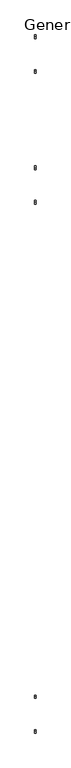
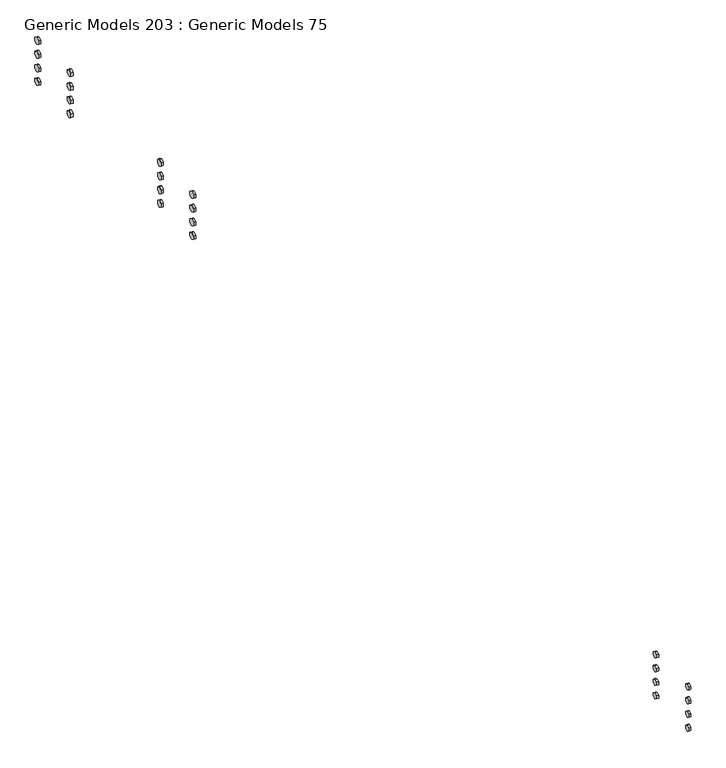
"""IFC4 building model written with IfcOpenShell, lengths in millimetres: proxy geometry, Generic Models 203 : Generic Models 75."""

from ifc_helpers import new_model, si_unit, frame, origin, place, context, project, spatial, polyline, outline, extrude, source, transform, mapped, element, save


def generic_models_203_generic_models_75_2103832a(model_context):
    return source(origin(), model_context, "Body", "SweptSolid", [
        extrude(outline(polyline([(30612.3964892, 271527.9099609), (30626.7031612, 271536.1699219), (30641.0098332, 271527.9099609), (30641.0098332, 271511.3900391), (30626.7031612, 271503.1300781), (30612.3964892, 271511.3900391), (30612.3964892, 271527.9099609)])), frame((31930.9715778, 0.0, 0.0), z_axis=(1.0, 0.0, 0.0), x_axis=(0.0, 1.0, 0.0)), (0.0, 0.0, 1.0), 11.90625),
        extrude(outline(polyline([(30612.3964892, 271604.1099609), (30626.7031612, 271612.3699219), (30641.0098332, 271604.1099609), (30641.0098332, 271587.5900391), (30626.7031612, 271579.3300781), (30612.3964892, 271587.5900391), (30612.3964892, 271604.1099609)])), frame((31930.9715778, 0.0, 0.0), z_axis=(1.0, 0.0, 0.0), x_axis=(0.0, 1.0, 0.0)), (0.0, 0.0, 1.0), 11.90625),
        extrude(outline(polyline([(30612.3964892, 271680.3099609), (30626.7031612, 271688.5699219), (30641.0098332, 271680.3099609), (30641.0098332, 271663.7900391), (30626.7031612, 271655.5300781), (30612.3964892, 271663.7900391), (30612.3964892, 271680.3099609)])), frame((31930.9715778, 0.0, 0.0), z_axis=(1.0, 0.0, 0.0), x_axis=(0.0, 1.0, 0.0)), (0.0, 0.0, 1.0), 11.90625),
        extrude(outline(polyline([(30612.3964892, 271756.5099609), (30626.7031612, 271764.7699219), (30641.0098332, 271756.5099609), (30641.0098332, 271739.9900391), (30626.7031612, 271731.7300781), (30612.3964892, 271739.9900391), (30612.3964892, 271756.5099609)])), frame((31930.9715778, 0.0, 0.0), z_axis=(1.0, 0.0, 0.0), x_axis=(0.0, 1.0, 0.0)), (0.0, 0.0, 1.0), 11.90625),
        extrude(outline(polyline([(30907.6714892, 271527.9099609), (30921.9781612, 271536.1699219), (30936.2848332, 271527.9099609), (30936.2848332, 271511.3900391), (30921.9781612, 271503.1300781), (30907.6714892, 271511.3900391), (30907.6714892, 271527.9099609)])), frame((31930.9715778, 0.0, 0.0), z_axis=(1.0, 0.0, 0.0), x_axis=(0.0, 1.0, 0.0)), (0.0, 0.0, 1.0), 11.90625),
        extrude(outline(polyline([(30907.6714892, 271604.1099609), (30921.9781612, 271612.3699219), (30936.2848332, 271604.1099609), (30936.2848332, 271587.5900391), (30921.9781612, 271579.3300781), (30907.6714892, 271587.5900391), (30907.6714892, 271604.1099609)])), frame((31930.9715778, 0.0, 0.0), z_axis=(1.0, 0.0, 0.0), x_axis=(0.0, 1.0, 0.0)), (0.0, 0.0, 1.0), 11.90625),
        extrude(outline(polyline([(30907.6714892, 271680.3099609), (30921.9781612, 271688.5699219), (30936.2848332, 271680.3099609), (30936.2848332, 271663.7900391), (30921.9781612, 271655.5300781), (30907.6714892, 271663.7900391), (30907.6714892, 271680.3099609)])), frame((31930.9715778, 0.0, 0.0), z_axis=(1.0, 0.0, 0.0), x_axis=(0.0, 1.0, 0.0)), (0.0, 0.0, 1.0), 11.90625),
        extrude(outline(polyline([(35158.6810781, 271681.575), (35158.6810781, 271662.525), (35142.1832942, 271653.0), (35125.6855103, 271662.525), (35125.6855103, 271681.575), (35142.1832942, 271691.1), (35158.6810781, 271681.575)])), frame((31930.9715778, 0.0, 0.0), z_axis=(1.0, 0.0, 0.0), x_axis=(0.0, 1.0, 0.0)), (0.0, 0.0, 1.0), 11.90625),
        extrude(outline(polyline([(35158.6810781, 271605.375), (35158.6810781, 271586.325), (35142.1832942, 271576.8), (35125.6855103, 271586.325), (35125.6855103, 271605.375), (35142.1832942, 271614.9), (35158.6810781, 271605.375)])), frame((31930.9715778, 0.0, 0.0), z_axis=(1.0, 0.0, 0.0), x_axis=(0.0, 1.0, 0.0)), (0.0, 0.0, 1.0), 11.90625),
        extrude(outline(polyline([(36571.5560781, 271529.175), (36571.5560781, 271510.125), (36555.0582942, 271500.6), (36538.5605103, 271510.125), (36538.5605103, 271529.175), (36555.0582942, 271538.7), (36571.5560781, 271529.175)])), frame((31930.9715778, 0.0, 0.0), z_axis=(1.0, 0.0, 0.0), x_axis=(0.0, 1.0, 0.0)), (0.0, 0.0, 1.0), 11.90625),
        extrude(outline(polyline([(36571.5560781, 271605.375), (36571.5560781, 271586.325), (36555.0582942, 271576.8), (36538.5605103, 271586.325), (36538.5605103, 271605.375), (36555.0582942, 271614.9), (36571.5560781, 271605.375)])), frame((31930.9715778, 0.0, 0.0), z_axis=(1.0, 0.0, 0.0), x_axis=(0.0, 1.0, 0.0)), (0.0, 0.0, 1.0), 11.90625),
        extrude(outline(polyline([(36571.5560781, 271681.575), (36571.5560781, 271662.525), (36555.0582942, 271653.0), (36538.5605103, 271662.525), (36538.5605103, 271681.575), (36555.0582942, 271691.1), (36571.5560781, 271681.575)])), frame((31930.9715778, 0.0, 0.0), z_axis=(1.0, 0.0, 0.0), x_axis=(0.0, 1.0, 0.0)), (0.0, 0.0, 1.0), 11.90625),
        extrude(outline(polyline([(36571.5560781, 271757.775), (36571.5560781, 271738.725), (36555.0582942, 271729.2), (36538.5605103, 271738.725), (36538.5605103, 271757.775), (36555.0582942, 271767.3), (36571.5560781, 271757.775)])), frame((31930.9715778, 0.0, 0.0), z_axis=(1.0, 0.0, 0.0), x_axis=(0.0, 1.0, 0.0)), (0.0, 0.0, 1.0), 11.90625),
        extrude(outline(polyline([(36276.2810781, 271529.175), (36276.2810781, 271510.125), (36259.7832942, 271500.6), (36243.2855103, 271510.125), (36243.2855103, 271529.175), (36259.7832942, 271538.7), (36276.2810781, 271529.175)])), frame((31930.9715778, 0.0, 0.0), z_axis=(1.0, 0.0, 0.0), x_axis=(0.0, 1.0, 0.0)), (0.0, 0.0, 1.0), 11.90625),
        extrude(outline(polyline([(36276.2810781, 271605.375), (36276.2810781, 271586.325), (36259.7832942, 271576.8), (36243.2855103, 271586.325), (36243.2855103, 271605.375), (36259.7832942, 271614.9), (36276.2810781, 271605.375)])), frame((31930.9715778, 0.0, 0.0), z_axis=(1.0, 0.0, 0.0), x_axis=(0.0, 1.0, 0.0)), (0.0, 0.0, 1.0), 11.90625),
        extrude(outline(polyline([(36276.2810781, 271681.575), (36276.2810781, 271662.525), (36259.7832942, 271653.0), (36243.2855103, 271662.525), (36243.2855103, 271681.575), (36259.7832942, 271691.1), (36276.2810781, 271681.575)])), frame((31930.9715778, 0.0, 0.0), z_axis=(1.0, 0.0, 0.0), x_axis=(0.0, 1.0, 0.0)), (0.0, 0.0, 1.0), 11.90625),
        extrude(outline(polyline([(36276.2810781, 271757.775), (36276.2810781, 271738.725), (36259.7832942, 271729.2), (36243.2855103, 271738.725), (36243.2855103, 271757.775), (36259.7832942, 271767.3), (36276.2810781, 271757.775)])), frame((31930.9715778, 0.0, 0.0), z_axis=(1.0, 0.0, 0.0), x_axis=(0.0, 1.0, 0.0)), (0.0, 0.0, 1.0), 11.90625),
        extrude(outline(polyline([(35453.9560781, 271529.175), (35453.9560781, 271510.125), (35437.4582942, 271500.6), (35420.9605103, 271510.125), (35420.9605103, 271529.175), (35437.4582942, 271538.7), (35453.9560781, 271529.175)])), frame((31930.9715778, 0.0, 0.0), z_axis=(1.0, 0.0, 0.0), x_axis=(0.0, 1.0, 0.0)), (0.0, 0.0, 1.0), 11.90625),
        extrude(outline(polyline([(35453.9560781, 271605.375), (35453.9560781, 271586.325), (35437.4582942, 271576.8), (35420.9605103, 271586.325), (35420.9605103, 271605.375), (35437.4582942, 271614.9), (35453.9560781, 271605.375)])), frame((31930.9715778, 0.0, 0.0), z_axis=(1.0, 0.0, 0.0), x_axis=(0.0, 1.0, 0.0)), (0.0, 0.0, 1.0), 11.90625),
        extrude(outline(polyline([(35453.9560781, 271681.575), (35453.9560781, 271662.525), (35437.4582942, 271653.0), (35420.9605103, 271662.525), (35420.9605103, 271681.575), (35437.4582942, 271691.1), (35453.9560781, 271681.575)])), frame((31930.9715778, 0.0, 0.0), z_axis=(1.0, 0.0, 0.0), x_axis=(0.0, 1.0, 0.0)), (0.0, 0.0, 1.0), 11.90625),
        extrude(outline(polyline([(35453.9560781, 271757.775), (35453.9560781, 271738.725), (35437.4582942, 271729.2), (35420.9605103, 271738.725), (35420.9605103, 271757.775), (35437.4582942, 271767.3), (35453.9560781, 271757.775)])), frame((31930.9715778, 0.0, 0.0), z_axis=(1.0, 0.0, 0.0), x_axis=(0.0, 1.0, 0.0)), (0.0, 0.0, 1.0), 11.90625),
        extrude(outline(polyline([(35158.6810781, 271529.175), (35158.6810781, 271510.125), (35142.1832942, 271500.6), (35125.6855103, 271510.125), (35125.6855103, 271529.175), (35142.1832942, 271538.7), (35158.6810781, 271529.175)])), frame((31930.9715778, 0.0, 0.0), z_axis=(1.0, 0.0, 0.0), x_axis=(0.0, 1.0, 0.0)), (0.0, 0.0, 1.0), 11.90625),
        extrude(outline(polyline([(35158.6810781, 271757.775), (35158.6810781, 271738.725), (35142.1832942, 271729.2), (35125.6855103, 271738.725), (35125.6855103, 271757.775), (35142.1832942, 271767.3), (35158.6810781, 271757.775)])), frame((31930.9715778, 0.0, 0.0), z_axis=(1.0, 0.0, 0.0), x_axis=(0.0, 1.0, 0.0)), (0.0, 0.0, 1.0), 11.90625),
        extrude(outline(polyline([(30907.6714892, 271756.5099609), (30921.9781612, 271764.7699219), (30936.2848332, 271756.5099609), (30936.2848332, 271739.9900391), (30921.9781612, 271731.7300781), (30907.6714892, 271739.9900391), (30907.6714892, 271756.5099609)])), frame((31930.9715778, 0.0, 0.0), z_axis=(1.0, 0.0, 0.0), x_axis=(0.0, 1.0, 0.0)), (0.0, 0.0, 1.0), 11.90625),
    ])


if __name__ == "__main__":
    model = new_model("IFC4")
    model_context = context("Model", 3, world=origin())
    ifc_project = project(units=[si_unit("LENGTHUNIT", "METRE", prefix="MILLI")], contexts=[model_context])
    site = spatial("IfcSite", under=ifc_project)
    building = spatial("IfcBuilding", under=site)
    placement = place(None, origin())
    generic_models_203_generic_models_75_shape = generic_models_203_generic_models_75_2103832a(model_context)
    element("IfcBuildingElementProxy", 1, Name="Generic Models 203 : Generic Models 75", ObjectType="Generic Models 203 : Generic Models 75", at=placement, inside=building, context=model_context, shape_type="MappedRepresentation", body=[
        mapped(generic_models_203_generic_models_75_shape, transform((0.0, 0.0, 0.0), x_axis=(1.0, 0.0, 0.0), y_axis=(0.0, 1.0, 0.0), z_axis=(0.0, 0.0, 1.0))),
    ])
    save(model, "model.ifc")

# Revit data of these elements
# Element 1 (IfcBuildingElementProxy, "Generic Models 203 : Generic Models 75")
#   Materials on its faces: "3/4\" DIA LAG BOLTS"
# Materials
#   "3/4\" DIA LAG BOLTS": class "Generic", colour RGB 255 255 0, transparency 0, Cost = 0
